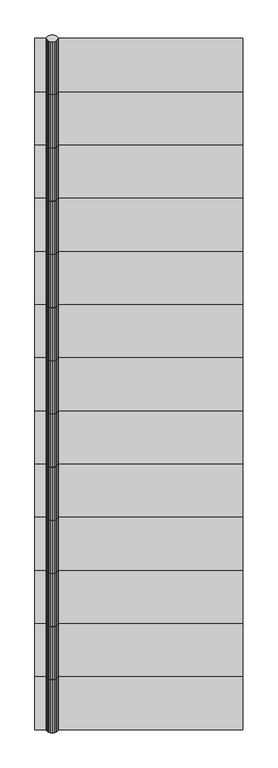
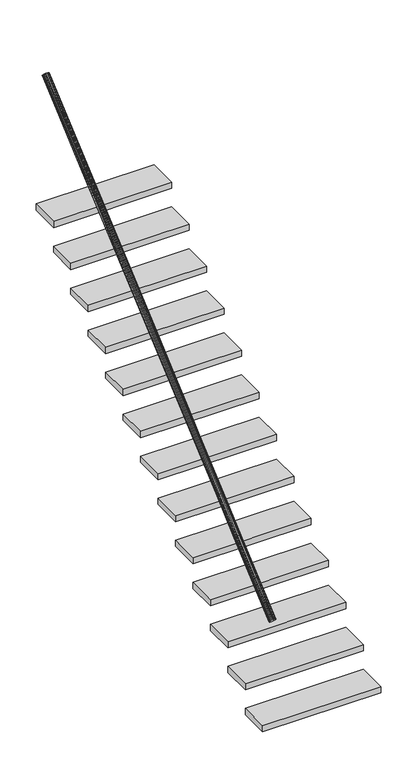
"""IFC4 building model written with IfcOpenShell, lengths in millimetres: stair geometry, 0_3d_modell."""

from ifc_helpers import new_model, si_unit, frame, origin, origin_with_axes, place, context, project, spatial, polyline, outline, extrude, source, transform, mapped, element, save


def stair_fbe942c3(model_context):
    return source(origin(), model_context, "Body", "SweptSolid", [
        extrude(outline(polyline([(1.2235871, -7.065663), (0.0, 0.0), (1.2235871, 7.0656631), (4.7745751, 13.4396898), (10.3053687, 18.498146), (17.2745751, 21.7458748), (25.0, 22.8649659), (32.7254249, 21.7458748), (39.6946313, 18.498146), (45.2254249, 13.4396898), (48.7764129, 7.0656631), (50.0, 0.0), (48.7764129, -7.065663), (45.2254249, -13.4396897), (39.6946313, -18.498146), (32.7254249, -21.7458748), (25.0, -22.8649659), (17.2745751, -21.7458748), (10.3053687, -18.498146), (4.7745751, -13.4396897), (1.2235871, -7.065663)])), frame((50.0, 934.9421971, 1663.8449509), z_axis=(0.0, 0.7569287102857108, 0.6534974579485451), x_axis=(1.0, 0.0, 0.0)), (0.0, 0.0, 1.0), 303.8595272),
        extrude(outline(polyline([(900.0, 474.9421971), (0.0, 474.9421971), (0.0, 704.9421971), (900.0, 704.9421971), (900.0, 474.9421971)])), frame((0.0, 0.0, 397.1428571), z_axis=(0.0, 0.0, 1.0), x_axis=(1.0, 0.0, 0.0)), (0.0, 0.0, 1.0), 50.0),
        extrude(outline(polyline([(1.2235871, -7.0656631), (0.0, 0.0), (1.2235871, 7.0656631), (4.7745751, 13.4396897), (10.3053687, 18.498146), (17.2745751, 21.7458748), (25.0, 22.8649659), (32.7254249, 21.7458748), (39.6946313, 18.498146), (45.2254249, 13.4396897), (48.7764129, 7.0656631), (50.0, 0.0), (48.7764129, -7.0656631), (45.2254249, -13.4396898), (39.6946313, -18.4981461), (32.7254249, -21.7458748), (25.0, -22.8649659), (17.2745751, -21.7458748), (10.3053687, -18.4981461), (4.7745751, -13.4396898), (1.2235871, -7.0656631)])), frame((50.0, 474.9421971, 1266.7020937), z_axis=(0.0, 0.7569287102857101, 0.653497457948546), x_axis=(1.0, 0.0, 0.0)), (0.0, 0.0, 1.0), 303.8595272),
        extrude(outline(polyline([(900.0, 704.9421971), (0.0, 704.9421971), (0.0, 934.9421971), (900.0, 934.9421971), (900.0, 704.9421971)])), frame((0.0, 0.0, 595.7142857), z_axis=(0.0, 0.0, 1.0), x_axis=(1.0, 0.0, 0.0)), (0.0, 0.0, 1.0), 50.0),
        extrude(outline(polyline([(900.0, 2314.9421971), (0.0, 2314.9421971), (0.0, 2544.9421971), (900.0, 2544.9421971), (900.0, 2314.9421971)])), frame((0.0, 0.0, 1985.7142857), z_axis=(0.0, 0.0, 1.0), x_axis=(1.0, 0.0, 0.0)), (0.0, 0.0, 1.0), 50.0),
        extrude(outline(polyline([(1.2235871, -7.065663), (0.0, 0.0), (1.2235871, 7.0656631), (4.7745751, 13.4396898), (10.3053687, 18.498146), (17.2745751, 21.7458748), (25.0, 22.8649659), (32.7254249, 21.7458748), (39.6946313, 18.498146), (45.2254249, 13.4396898), (48.7764129, 7.0656631), (50.0, 0.0), (48.7764129, -7.065663), (45.2254249, -13.4396897), (39.6946313, -18.498146), (32.7254249, -21.7458748), (25.0, -22.8649659), (17.2745751, -21.7458748), (10.3053687, -18.498146), (4.7745751, -13.4396897), (1.2235871, -7.065663)])), frame((50.0, 1164.9421971, 1862.4163795), z_axis=(0.0, 0.7569287102857027, 0.6534974579485544), x_axis=(1.0, 0.0, 0.0)), (0.0, 0.0, 1.0), 303.8595272),
        extrude(outline(polyline([(900.0, 1394.9421971), (0.0, 1394.9421971), (0.0, 1624.9421971), (900.0, 1624.9421971), (900.0, 1394.9421971)])), frame((0.0, 0.0, 1191.4285714), z_axis=(0.0, 0.0, 1.0), x_axis=(1.0, 0.0, 0.0)), (0.0, 0.0, 1.0), 50.0),
        extrude(outline(polyline([(900.0, 1164.9421971), (0.0, 1164.9421971), (0.0, 1394.9421971), (900.0, 1394.9421971), (900.0, 1164.9421971)])), frame((0.0, 0.0, 992.8571429), z_axis=(0.0, 0.0, 1.0), x_axis=(1.0, 0.0, 0.0)), (0.0, 0.0, 1.0), 50.0),
        extrude(outline(polyline([(900.0, 1624.9421971), (0.0, 1624.9421971), (0.0, 1854.9421971), (900.0, 1854.9421971), (900.0, 1624.9421971)])), frame((0.0, 0.0, 1390.0), z_axis=(0.0, 0.0, 1.0), x_axis=(1.0, 0.0, 0.0)), (0.0, 0.0, 1.0), 50.0),
        extrude(outline(polyline([(900.0, 2774.9421971), (0.0, 2774.9421971), (0.0, 3004.9421971), (900.0, 3004.9421971), (900.0, 2774.9421971)])), frame((0.0, 0.0, 2382.8571429), z_axis=(0.0, 0.0, 1.0), x_axis=(1.0, 0.0, 0.0)), (0.0, 0.0, 1.0), 50.0),
        extrude(outline(polyline([(1.2235871, -7.065663), (0.0, 0.0), (1.2235871, 7.0656631), (4.7745751, 13.4396898), (10.3053687, 18.498146), (17.2745751, 21.7458748), (25.0, 22.8649659), (32.7254249, 21.7458748), (39.6946313, 18.498146), (45.2254249, 13.4396898), (48.7764129, 7.0656631), (50.0, 0.0), (48.7764129, -7.065663), (45.2254249, -13.4396897), (39.6946313, -18.498146), (32.7254249, -21.7458748), (25.0, -22.8649659), (17.2745751, -21.7458748), (10.3053687, -18.498146), (4.7745751, -13.4396897), (1.2235871, -7.065663)])), frame((50.0, 2544.9421971, 3053.8449509), z_axis=(0.0, 0.756928710285712, 0.6534974579485439), x_axis=(1.0, 0.0, 0.0)), (0.0, 0.0, 1.0), 303.8595272),
        extrude(outline(polyline([(1.2235871, -7.065663), (0.0, 0.0), (1.2235871, 7.0656631), (4.7745751, 13.4396897), (10.3053687, 18.498146), (17.2745751, 21.7458748), (25.0, 22.8649659), (32.7254249, 21.7458748), (39.6946313, 18.498146), (45.2254249, 13.4396897), (48.7764129, 7.0656631), (50.0, 0.0), (48.7764129, -7.065663), (45.2254249, -13.4396897), (39.6946313, -18.498146), (32.7254249, -21.7458748), (25.0, -22.8649659), (17.2745751, -21.7458748), (10.3053687, -18.498146), (4.7745751, -13.4396897), (1.2235871, -7.065663)])), frame((50.0, 14.9421971, 869.5592366), z_axis=(0.0, 0.7569287102857073, 0.6534974579485493), x_axis=(1.0, 0.0, 0.0)), (0.0, 0.0, 1.0), 303.8595272),
        extrude(outline(polyline([(1.2235871, -7.065663), (0.0, 0.0), (1.2235871, 7.0656631), (4.7745751, 13.4396898), (10.3053687, 18.498146), (17.2745751, 21.7458748), (25.0, 22.8649659), (32.7254249, 21.7458748), (39.6946313, 18.498146), (45.2254249, 13.4396898), (48.7764129, 7.0656631), (50.0, 0.0), (48.7764129, -7.065663), (45.2254249, -13.4396897), (39.6946313, -18.498146), (32.7254249, -21.7458748), (25.0, -22.8649659), (17.2745751, -21.7458748), (10.3053687, -18.498146), (4.7745751, -13.4396897), (1.2235871, -7.065663)])), frame((50.0, 244.9421971, 1068.1306652), z_axis=(0.0, 0.7569287102856902, 0.6534974579485691), x_axis=(1.0, 0.0, 0.0)), (0.0, 0.0, 1.0), 303.8595272),
        extrude(outline(polyline([(1.2235871, -7.065663), (0.0, 0.0), (1.2235871, 7.0656631), (4.7745751, 13.4396897), (10.3053687, 18.498146), (17.2745751, 21.7458748), (25.0, 22.8649659), (32.7254249, 21.7458748), (39.6946313, 18.498146), (45.2254249, 13.4396897), (48.7764129, 7.0656631), (50.0, 0.0), (48.7764129, -7.065663), (45.2254249, -13.4396898), (39.6946313, -18.498146), (32.7254249, -21.7458748), (25.0, -22.8649659), (17.2745751, -21.7458748), (10.3053687, -18.498146), (4.7745751, -13.4396898), (1.2235871, -7.065663)])), frame((50.0, 704.9421971, 1465.2735223), z_axis=(0.0, 0.7569287102857122, 0.6534974579485435), x_axis=(1.0, 0.0, 0.0)), (0.0, 0.0, 1.0), 303.8595272),
        extrude(outline(polyline([(1.2235871, -7.065663), (0.0, 0.0), (1.2235871, 7.0656631), (4.7745751, 13.4396898), (10.3053687, 18.498146), (17.2745751, 21.7458748), (25.0, 22.8649659), (32.7254249, 21.7458748), (39.6946313, 18.498146), (45.2254249, 13.4396898), (48.7764129, 7.0656631), (50.0, 0.0), (48.7764129, -7.065663), (45.2254249, -13.4396897), (39.6946313, -18.498146), (32.7254249, -21.7458748), (25.0, -22.8649659), (17.2745751, -21.7458748), (10.3053687, -18.498146), (4.7745751, -13.4396897), (1.2235871, -7.065663)])), frame((50.0, 2774.9421971, 3252.4163795), z_axis=(0.0, 0.7569287102857426, 0.6534974579485083), x_axis=(1.0, 0.0, 0.0)), (0.0, 0.0, 1.0), 303.8595272),
        extrude(outline(polyline([(900.0, 244.9421971), (0.0, 244.9421971), (0.0, 474.9421971), (900.0, 474.9421971), (900.0, 244.9421971)])), frame((0.0, 0.0, 198.5714286), z_axis=(0.0, 0.0, 1.0), x_axis=(1.0, 0.0, 0.0)), (0.0, 0.0, 1.0), 50.0),
        extrude(outline(polyline([(1.2235871, -7.065663), (0.0, 0.0), (1.2235871, 7.0656631), (4.7745751, 13.4396898), (10.3053687, 18.498146), (17.2745751, 21.7458748), (25.0, 22.8649659), (32.7254249, 21.7458748), (39.6946313, 18.498146), (45.2254249, 13.4396898), (48.7764129, 7.0656631), (50.0, 0.0), (48.7764129, -7.065663), (45.2254249, -13.4396897), (39.6946313, -18.498146), (32.7254249, -21.7458748), (25.0, -22.8649659), (17.2745751, -21.7458748), (10.3053687, -18.498146), (4.7745751, -13.4396897), (1.2235871, -7.065663)])), frame((50.0, 1854.9421971, 2458.1306652), z_axis=(0.0, 0.7569287102857091, 0.6534974579485472), x_axis=(1.0, 0.0, 0.0)), (0.0, 0.0, 1.0), 303.8595272),
        extrude(outline(polyline([(900.0, 934.9421971), (0.0, 934.9421971), (0.0, 1164.9421971), (900.0, 1164.9421971), (900.0, 934.9421971)])), frame((0.0, 0.0, 794.2857143), z_axis=(0.0, 0.0, 1.0), x_axis=(1.0, 0.0, 0.0)), (0.0, 0.0, 1.0), 50.0),
        extrude(outline(polyline([(1.2235871, -7.065663), (0.0, 0.0), (1.2235871, 7.0656631), (4.7745751, 13.4396897), (10.3053687, 18.498146), (17.2745751, 21.7458748), (25.0, 22.8649659), (32.7254249, 21.7458748), (39.6946313, 18.498146), (45.2254249, 13.4396897), (48.7764129, 7.0656631), (50.0, 0.0), (48.7764129, -7.065663), (45.2254249, -13.4396897), (39.6946313, -18.498146), (32.7254249, -21.7458748), (25.0, -22.8649659), (17.2745751, -21.7458748), (10.3053687, -18.498146), (4.7745751, -13.4396897), (1.2235871, -7.065663)])), frame((50.0, 1624.9421971, 2259.5592366), z_axis=(0.0, 0.7569287102856798, 0.6534974579485812), x_axis=(1.0, 0.0, 0.0)), (0.0, 0.0, 1.0), 303.8595272),
        extrude(outline(polyline([(1.2235871, -7.0656631), (0.0, 0.0), (1.2235871, 7.0656631), (4.7745751, 13.4396897), (10.3053687, 18.498146), (17.2745751, 21.7458748), (25.0, 22.8649659), (32.7254249, 21.7458748), (39.6946313, 18.498146), (45.2254249, 13.4396897), (48.7764129, 7.0656631), (50.0, 0.0), (48.7764129, -7.0656631), (45.2254249, -13.4396898), (39.6946313, -18.498146), (32.7254249, -21.7458748), (25.0, -22.8649659), (17.2745751, -21.7458748), (10.3053687, -18.498146), (4.7745751, -13.4396898), (1.2235871, -7.0656631)])), frame((50.0, 1394.9421971, 2060.987808), z_axis=(0.0, 0.7569287102856966, 0.6534974579485615), x_axis=(1.0, 0.0, 0.0)), (0.0, 0.0, 1.0), 303.8595272),
        extrude(outline(polyline([(900.0, 2544.9421971), (0.0, 2544.9421971), (0.0, 2774.9421971), (900.0, 2774.9421971), (900.0, 2544.9421971)])), frame((0.0, 0.0, 2184.2857143), z_axis=(0.0, 0.0, 1.0), x_axis=(1.0, 0.0, 0.0)), (0.0, 0.0, 1.0), 50.0),
        extrude(outline(polyline([(900.0, 14.9421971), (0.0, 14.9421971), (0.0, 244.9421971), (900.0, 244.9421971), (900.0, 14.9421971)])), origin_with_axes(), (0.0, 0.0, 1.0), 50.0),
        extrude(outline(polyline([(900.0, 1854.9421971), (0.0, 1854.9421971), (0.0, 2084.9421971), (900.0, 2084.9421971), (900.0, 1854.9421971)])), frame((0.0, 0.0, 1588.5714286), z_axis=(0.0, 0.0, 1.0), x_axis=(1.0, 0.0, 0.0)), (0.0, 0.0, 1.0), 50.0),
        extrude(outline(polyline([(1.2235871, -7.0656631), (0.0, 0.0), (1.2235871, 7.0656631), (4.7745751, 13.4396897), (10.3053687, 18.498146), (17.2745751, 21.7458748), (25.0, 22.8649659), (32.7254249, 21.7458748), (39.6946313, 18.498146), (45.2254249, 13.4396897), (48.7764129, 7.0656631), (50.0, 0.0), (48.7764129, -7.0656631), (45.2254249, -13.4396898), (39.6946313, -18.4981461), (32.7254249, -21.7458748), (25.0, -22.8649659), (17.2745751, -21.7458748), (10.3053687, -18.4981461), (4.7745751, -13.4396898), (1.2235871, -7.0656631)])), frame((50.0, 2084.9421971, 2656.7020937), z_axis=(0.0, 0.7569287102856974, 0.6534974579485607), x_axis=(1.0, 0.0, 0.0)), (0.0, 0.0, 1.0), 303.8595272),
        extrude(outline(polyline([(1.2235871, -7.065663), (0.0, 0.0), (1.2235871, 7.0656631), (4.7745751, 13.4396897), (10.3053687, 18.498146), (17.2745751, 21.7458748), (25.0, 22.8649659), (32.7254249, 21.7458748), (39.6946313, 18.498146), (45.2254249, 13.4396897), (48.7764129, 7.0656631), (50.0, 0.0), (48.7764129, -7.065663), (45.2254249, -13.4396898), (39.6946313, -18.498146), (32.7254249, -21.7458748), (25.0, -22.8649659), (17.2745751, -21.7458748), (10.3053687, -18.498146), (4.7745751, -13.4396898), (1.2235871, -7.065663)])), frame((50.0, 2314.9421971, 2855.2735223), z_axis=(0.0, 0.756928710285704, 0.653497457948553), x_axis=(1.0, 0.0, 0.0)), (0.0, 0.0, 1.0), 303.8595272),
        extrude(outline(polyline([(900.0, 2084.9421971), (0.0, 2084.9421971), (0.0, 2314.9421971), (900.0, 2314.9421971), (900.0, 2084.9421971)])), frame((0.0, 0.0, 1787.1428571), z_axis=(0.0, 0.0, 1.0), x_axis=(1.0, 0.0, 0.0)), (0.0, 0.0, 1.0), 50.0),
    ])


if __name__ == "__main__":
    model = new_model("IFC4")
    model_context = context("Model", 3, world=origin())
    ifc_project = project(units=[si_unit("LENGTHUNIT", "METRE", prefix="MILLI")], contexts=[model_context])
    site = spatial("IfcSite", under=ifc_project)
    building = spatial("IfcBuilding", under=site)
    placement = place(None, origin())
    stair_shape = stair_fbe942c3(model_context)
    element("IfcStair", 1, ObjectType="0_3d_modell", at=placement, inside=building, context=model_context, shape_type="MappedRepresentation", body=[
        mapped(stair_shape, transform((0.0, 0.0, 0.0), x_axis=(1.0, 0.0, 0.0), y_axis=(0.0, 1.0, 0.0), z_axis=(0.0, 0.0, 1.0))),
    ])
    save(model, "model.ifc")

# Revit data of these elements
# Element 1 (IfcStair, "0_3d_modell")
#   Materials on its faces: "*1", "weiss"
# Materials
#   "*1": class "Unassigned", colour RGB 175 175 175, transparency 0
#   "weiss": class "Unassigned", colour RGB 255 255 255, transparency 0
